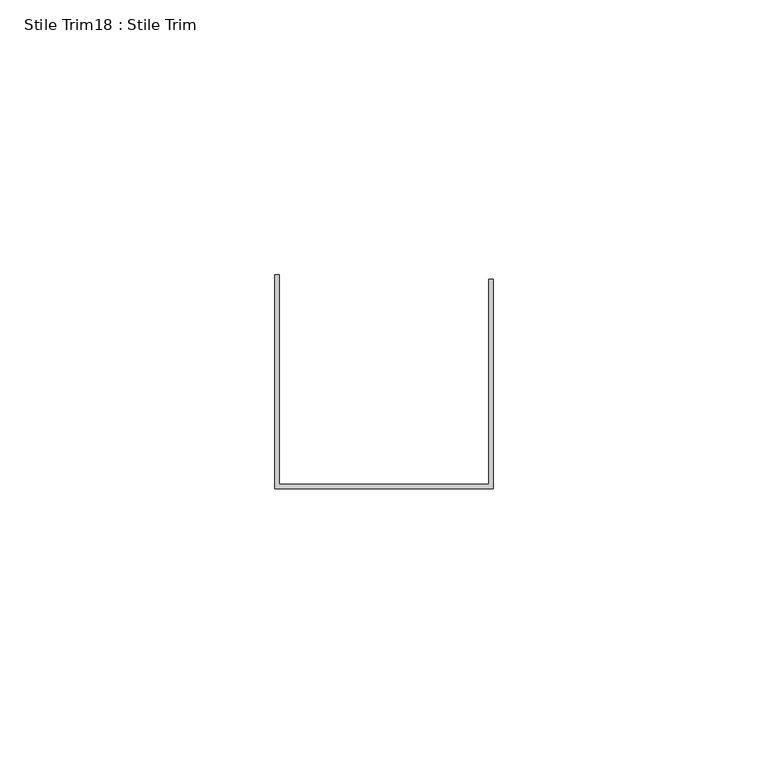
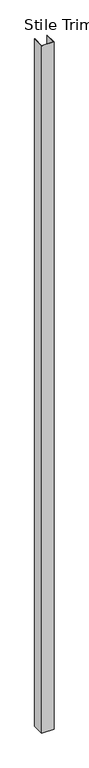
"""IFC4 building model written with IfcOpenShell, lengths in millimetres: proxy geometry, Stile Trim18 : Stile Trim."""

from ifc_helpers import new_model, si_unit, frame, origin, place, context, project, spatial, polyline, outline, extrude, source, transform, mapped, element, save


def stile_trim18_stile_trim_de7d98ae(model_context):
    return source(origin(), model_context, "Body", "SweptSolid", [
        extrude(outline(polyline([(587327.0060739, -533978.3912841), (587327.0060739, -533939.5038841), (587327.7934739, -533939.5038841), (587327.7934739, -533977.6038841), (587365.8934739, -533977.6038841), (587365.8934739, -533940.2912841), (587366.6808739, -533940.2912841), (587366.6808739, -533978.3912841), (587327.0060739, -533978.3912841)])), frame((0.0, 0.0, 50.8), z_axis=(0.0, 0.0, 1.0), x_axis=(1.0, 0.0, 0.0)), (0.0, 0.0, 1.0), 2350.3929688),
    ])


if __name__ == "__main__":
    model = new_model("IFC4")
    model_context = context("Model", 3, world=origin())
    ifc_project = project(units=[si_unit("LENGTHUNIT", "METRE", prefix="MILLI")], contexts=[model_context])
    site = spatial("IfcSite", under=ifc_project)
    building = spatial("IfcBuilding", under=site)
    placement = place(None, origin())
    stile_trim18_stile_trim_shape = stile_trim18_stile_trim_de7d98ae(model_context)
    element("IfcBuildingElementProxy", 1, Name="Stile Trim18 : Stile Trim", ObjectType="Stile Trim18 : Stile Trim", at=placement, inside=building, context=model_context, shape_type="MappedRepresentation", body=[
        mapped(stile_trim18_stile_trim_shape, transform((0.0, 0.0, 0.0), x_axis=(1.0, 0.0, 0.0), y_axis=(0.0, 1.0, 0.0), z_axis=(0.0, 0.0, 1.0))),
    ])
    save(model, "model.ifc")

# Revit data of these elements
# Element 1 (IfcBuildingElementProxy, "Stile Trim18 : Stile Trim")
#   Materials on its faces: "EDGE TRIM BY MTL PANEL MFR."
# Materials
#   "EDGE TRIM BY MTL PANEL MFR.": class "Generic", colour RGB 239 242 240, transparency 0, Cost = 0
